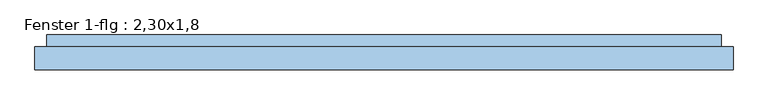
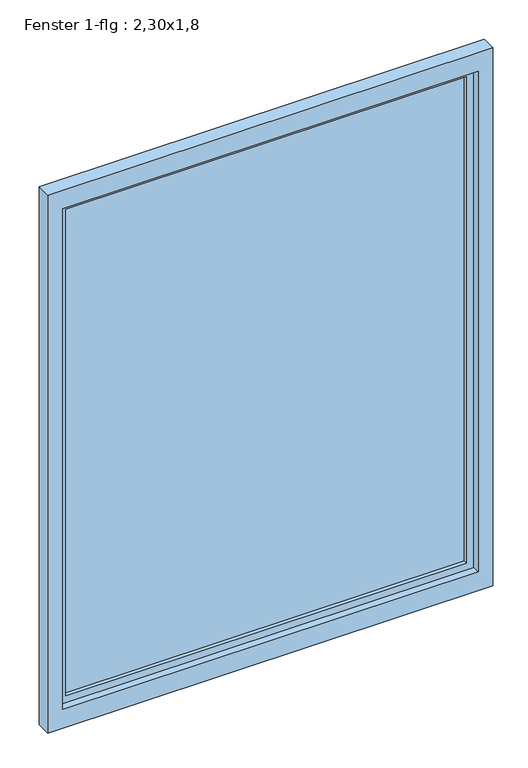
"""IFC4 building model written with IfcOpenShell, lengths in millimetres: window geometry, Fenster 1-flg : 2,30x1,8."""

from ifc_helpers import new_model, si_unit, frame, origin, place, context, project, spatial, polyline, outline, extrude, faceted_brep, source, transform, mapped, element, save


def fenster_1_flg_2_30x1_8_c8530eb6(model_context):
    return source(origin(), model_context, "Body", "SolidModel", [
        extrude(outline(polyline([(3300.0, 900.0), (3300.0, -900.0), (1000.0, -900.0), (1000.0, 900.0), (3300.0, 900.0)]), holes=[polyline([(3220.0, 840.0), (1080.0, 840.0), (1080.0, -840.0), (3220.0, -840.0), (3220.0, 840.0)])]), frame((0.0, -5.0, 0.0), z_axis=(0.0, 1.0, 0.0), x_axis=(0.0, 0.0, 1.0)), (0.0, 0.0, 1.0), 60.0),
        faceted_brep([(870.0, 55.0, 3250.0), (870.0, 55.0, 1050.0), (870.0, 85.0, 1050.0), (870.0, 85.0, 3250.0), (-870.0, 85.0, 1050.0), (-870.0, 85.0, 3250.0), (810.0, 85.0, 1110.0), (810.0, 85.0, 3190.0), (-810.0, 85.0, 3190.0), (-810.0, 85.0, 1110.0), (-870.0, 55.0, 1050.0), (-870.0, 55.0, 3250.0), (840.0, 55.0, 3220.0), (840.0, 55.0, 1080.0), (-840.0, 55.0, 1080.0), (-840.0, 55.0, 3220.0), (840.0, 25.0, 3220.0), (840.0, 25.0, 1080.0), (-840.0, 25.0, 1080.0), (-840.0, 25.0, 3220.0), (810.0, 25.0, 3190.0), (810.0, 25.0, 1110.0), (-810.0, 25.0, 1110.0), (-810.0, 25.0, 3190.0)], [[[0, 1, 2, 3]], [[3, 2, 4, 5], [6, 7, 8, 9]], [[1, 10, 4, 2]], [[1, 0, 11, 10], [12, 13, 14, 15]], [[16, 17, 13, 12]], [[17, 18, 14, 13]], [[17, 16, 19, 18], [20, 21, 22, 23]], [[7, 6, 21, 20]], [[6, 9, 22, 21]], [[10, 11, 5, 4]], [[18, 19, 15, 14]], [[9, 8, 23, 22]], [[11, 0, 3, 5]], [[19, 16, 12, 15]], [[8, 7, 20, 23]]]),
        extrude(outline(polyline([(810.0, 70.0), (810.0, 40.0), (-810.0, 40.0), (-810.0, 70.0), (810.0, 70.0)])), frame((0.0, 0.0, 1110.0), z_axis=(0.0, 0.0, 1.0), x_axis=(1.0, 0.0, 0.0)), (0.0, 0.0, 1.0), 2080.0),
    ])


if __name__ == "__main__":
    model = new_model("IFC4")
    model_context = context("Model", 3, world=origin())
    ifc_project = project(units=[si_unit("LENGTHUNIT", "METRE", prefix="MILLI")], contexts=[model_context])
    site = spatial("IfcSite", under=ifc_project)
    building = spatial("IfcBuilding", under=site)
    placement = place(None, origin())
    fenster_1_flg_2_30x1_8_shape = fenster_1_flg_2_30x1_8_c8530eb6(model_context)
    element("IfcWindow", 1, ObjectType="Fenster 1-flg : 2,30x1,8", at=placement, inside=building, context=model_context, shape_type="MappedRepresentation", body=[
        mapped(fenster_1_flg_2_30x1_8_shape, transform((0.0, 0.0, 0.0), x_axis=(1.0, 0.0, 0.0), y_axis=(0.0, 1.0, 0.0), z_axis=(0.0, 0.0, 1.0))),
    ])
    save(model, "model.ifc")

# Revit data of these elements
# Type "Fenster 1-flg : 2,30x1,8"
#   Type Mark = "71"
#   Operation = "SinglePanel"
#   Keynote = "16.05.01"
#   Visual Light Transmittance = 0.9
#   Solar Heat Gain Coefficient = 0.86
#   Rough Width = 1.800 m
#   Rough Height = 2.300 m
#   Heat Transfer Coefficient (U) = 5.5617 W/(m²·K)
#   Rahmentiefe = 0.060 m
#   Rahmenhöhe - unten = 0.080 m
#   Rahmenhöhe - oben = 0.080 m
#   Rahmenbreite = 0.060 m
#   Height = 2.300 m
#   Tiefe Flügel = 0.060 m
#   Flügelbreite = 0.060 m
#   Einbautiefe (von außen) [instance default] = 0.100 m
#   Width = 1.800 m
#   Klappflügel [instance default] = no
#   Kippflügel [instance default] = yes
#   Öffnungsrichtung in Draufsicht anzeigen [instance default] = no
#   Drehflügel 1 [instance default] = yes
#   Rahmen 1 [instance default] = none
#   Glas [instance default] = none
#   Flügel [instance default] = none
#   Fensterbank Innenseite [instance default] = none
#   Fensterbank Außenseite [instance default] = none
#   Construction Type Id = ""
#   Wall Closure = (empty or 0)
#   Analytic Construction = (empty or 0)
# Element 1 (IfcWindow, "Fenster 1-flg : 2,30x1,8")
#   Einbautiefe (von außen) = 0.220 m
#   Materials on its faces: "Kunststoff - Weiß", "Glas"
# Materials
#   "Kunststoff - Weiß": class "Kunststoff", colour RGB 249 249 249, transparency 0, Cost = 0
#   "Glas": class "Glas", colour RGB 0 0 255, transparency 0.75, Comments = "Render-Darstellung nicht aktualisiert ", Cost = 0
